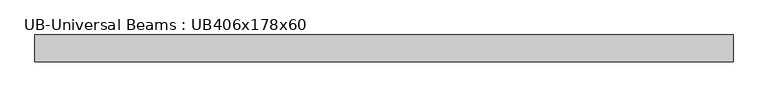
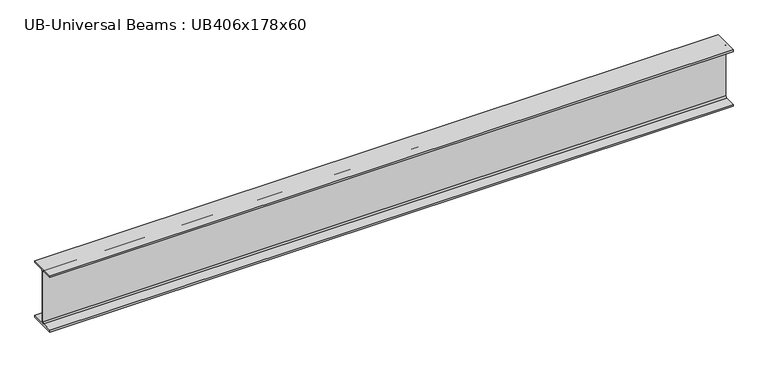
"""IFC4 building model written with IfcOpenShell, lengths in millimetres: beam geometry, UB-Universal Beams : UB406x178x60."""

from ifc_helpers import new_model, si_unit, point, frame, frame_2d, origin, place, context, project, spatial, polyline, circle_curve, trimmed, segment, composite_curve, outline, extrude, source, transform, mapped, element, save


def ub_universal_beams_ub406x178x60_0db8b4c4(model_context):
    return source(origin(), model_context, "Body", "SweptSolid", [
        extrude(outline(composite_curve([segment(polyline([(88.95, -190.4), (88.95, -203.2), (-88.95, -203.2), (-88.95, -190.4), (-14.15, -190.4)]), True, "CONTINUOUS"), segment(trimmed(circle_curve(frame_2d((-14.15, -180.2)), 10.2), [point((-14.15, -190.4))], [point((-3.95, -180.2))], True, "CARTESIAN"), True, "CONTINUOUS"), segment(polyline([(-3.95, -180.2), (-3.95, 180.2)]), True, "CONTINUOUS"), segment(trimmed(circle_curve(frame_2d((-14.15, 180.2)), 10.2), [point((-3.95, 180.2))], [point((-14.15, 190.4))], True, "CARTESIAN"), True, "CONTINUOUS"), segment(polyline([(-14.15, 190.4), (-88.95, 190.4), (-88.95, 203.2), (88.95, 203.2), (88.95, 190.4), (14.15, 190.4)]), True, "CONTINUOUS"), segment(trimmed(circle_curve(frame_2d((14.15, 180.2)), 10.2), [point((14.15, 190.4))], [point((3.95, 180.2))], True, "CARTESIAN"), True, "CONTINUOUS"), segment(polyline([(3.95, 180.2), (3.95, -180.2)]), True, "CONTINUOUS"), segment(trimmed(circle_curve(frame_2d((14.15, -180.2)), 10.2), [point((3.95, -180.2))], [point((14.15, -190.4))], True, "CARTESIAN"), True, "CONTINUOUS"), segment(polyline([(14.15, -190.4), (88.95, -190.4)]), True, "CONTINUOUS")], self_intersect=False)), frame((-2352.35, 0.0, 0.0), z_axis=(1.0, 0.0, 0.0), x_axis=(0.0, 1.0, 0.0)), (0.0, 0.0, 1.0), 4653.7),
    ])


if __name__ == "__main__":
    model = new_model("IFC4")
    model_context = context("Model", 3, world=origin())
    ifc_project = project(units=[si_unit("LENGTHUNIT", "METRE", prefix="MILLI")], contexts=[model_context])
    site = spatial("IfcSite", under=ifc_project)
    building = spatial("IfcBuilding", under=site)
    placement = place(None, origin())
    ub_universal_beams_ub406x178x60_shape = ub_universal_beams_ub406x178x60_0db8b4c4(model_context)
    element("IfcBeam", 1, ObjectType="UB-Universal Beams : UB406x178x60", at=placement, inside=building, context=model_context, shape_type="MappedRepresentation", body=[
        mapped(ub_universal_beams_ub406x178x60_shape, transform((0.0, 0.0, 0.0), x_axis=(1.0, 0.0, 0.0), y_axis=(0.0, 1.0, 0.0), z_axis=(0.0, 0.0, 1.0))),
    ])
    save(model, "model.ifc")

# Revit data of these elements
# Type "UB-Universal Beams : UB406x178x60"
#   Section Name Key = "UB406X178X60"
#   Width = 17.79 cm
#   Web Thickness = 0.79 cm
#   Web Fillet = 1.02 cm
#   Warping Constant = 466000.0 cm⁶
#   Torsional Moment of Inertia = 33.30 cm⁴
#   Section Area = 76.5 cm²
#   Plastic Modulus weak axis = 209.0 cm³
#   Plastic Modulus strong axis = 1200.0 cm³
#   Nominal Weight = 60.0998 kgf/m
#   Moment of Inertia weak axis = 1203.00 cm⁴
#   Moment of Inertia strong axis = 21596.00 cm⁴
#   Height = 40.64 cm
#   Flange Thickness = 1.28 cm
#   Elastic Modulus weak axis = 135.0 cm³
#   Elastic Modulus strong axis = 1063.0 cm³
#   Centroid Vertical = 20.32 cm
#   Centroid Horizontal = 8.895 cm
#   Bolt Spacing = 9.0 cm
#   Length [instance default] = 1500 mm
#   Structural Material [instance default] = Metal - Steel 43-275
#   Type Comments = ""
#   Assembly Code = ""
# Element 1 (IfcBeam, "UB-Universal Beams : UB406x178x60")
#   Materials on its faces: "Metal - Steel 43-275"
# Materials
#   "Metal - Steel 43-275": class "Metal", colour RGB 247 247 247, transparency 0, Cost = 0
